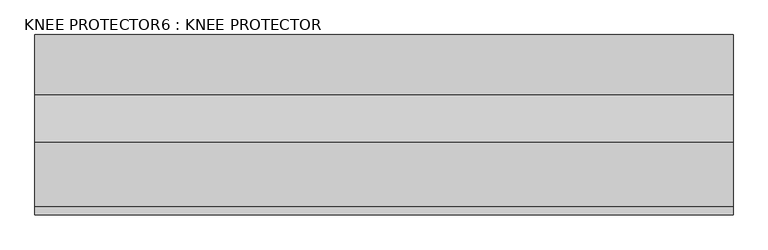
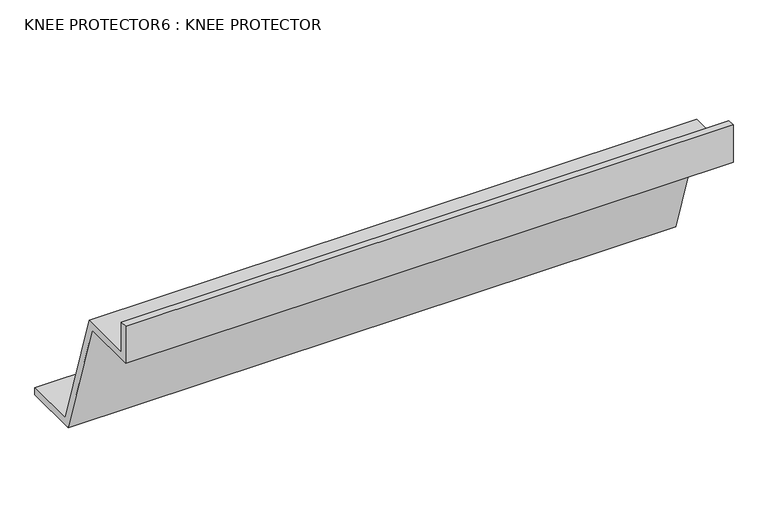
"""IFC4 building model written with IfcOpenShell, lengths in millimetres: furniture geometry, KNEE PROTECTOR6 : KNEE PROTECTOR."""

import ifcopenshell
import ifcopenshell.guid

model = None  # the IFC model being written
_history = None  # IfcOwnerHistory: only IFC2X3 demands one
_inside = {}  # id of a spatial element -> (the spatial element, [elements in it])
_under = {}  # id of a project, library or spatial element -> (it, [spatial elements below it])
_declared = {}  # id of a project -> (the project, [libraries it declares])
_typed = {}  # id of a type object -> (the type object, [elements of that type])
_made_of = {}  # id of a material, layer set ... -> (it, [elements and type objects made of it])


def new_model(schema):
    """Start an empty IFC model of exactly this schema.

    Asked for "IFC4X3", IfcOpenShell would pick the latest addendum, in which some entities
    have other attributes; the version numbers below select the first issue.
    IFC2X3 requires an IfcOwnerHistory on every rooted entity: one is made here for all.
    """
    global model, _history
    if schema == "IFC4X3":
        model = ifcopenshell.file(schema_version=(4, 3, 0, 0))
    else:
        model = ifcopenshell.file(schema=schema)
    _inside.clear()
    _under.clear()
    _declared.clear()
    _typed.clear()
    _made_of.clear()
    _history = None
    if model.schema == "IFC2X3":
        org = make("IfcOrganization", Name="unknown")
        user = make(
            "IfcPersonAndOrganization",
            ThePerson=make("IfcPerson", FamilyName="unknown"),
            TheOrganization=org,
        )
        app = make(
            "IfcApplication",
            ApplicationDeveloper=org,
            Version="unknown",
            ApplicationFullName="unknown",
            ApplicationIdentifier="unknown",
        )
        _history = make(
            "IfcOwnerHistory",
            OwningUser=user,
            OwningApplication=app,
            ChangeAction="ADDED",
            CreationDate=0,
        )
    return model


def make(cls, **values):
    """One entity of the class cls with the attributes given. An attribute that is None is left unset."""
    return model.create_entity(
        cls, **{name: value for name, value in values.items() if value is not None}
    )


def rooted(cls, **values):
    """An entity with a GlobalId (a new one), such as an element, a storey or a relation."""
    return make(cls, GlobalId=ifcopenshell.guid.new(), OwnerHistory=_history, **values)


def si_unit(unit_type, name, prefix=None):
    """IfcSIUnit, for example si_unit("LENGTHUNIT", "METRE", prefix="MILLI")."""
    return make("IfcSIUnit", UnitType=unit_type, Prefix=prefix, Name=name)


def assignment(units):
    """IfcUnitAssignment: the units of a project."""
    return None if units is None else make("IfcUnitAssignment", Units=units)


def point(xyz):
    """IfcCartesianPoint."""
    return None if xyz is None else make("IfcCartesianPoint", Coordinates=xyz)


def direction(xyz):
    """IfcDirection."""
    return None if xyz is None else make("IfcDirection", DirectionRatios=xyz)


def frame(location, z_axis=None, x_axis=None):
    """IfcAxis2Placement3D, a coordinate frame: its origin and axes. An axis left out is left unset."""
    return make(
        "IfcAxis2Placement3D",
        Location=point(location),
        Axis=direction(z_axis),
        RefDirection=direction(x_axis),
    )


def origin():
    """The frame at (0, 0, 0) with its axes left unset."""
    return frame((0.0, 0.0, 0.0))


def place(relative_to, where):
    """IfcLocalPlacement: puts the frame where relative to a parent placement (None: the world)."""
    return make(
        "IfcLocalPlacement", PlacementRelTo=relative_to, RelativePlacement=where
    )


def context(
    kind, dimensions, precision=None, world=None, true_north=None, identifier=None
):
    """IfcGeometricRepresentationContext, for example the 3D "Model" context."""
    return make(
        "IfcGeometricRepresentationContext",
        ContextIdentifier=identifier,
        ContextType=kind,
        CoordinateSpaceDimension=dimensions,
        Precision=precision,
        WorldCoordinateSystem=world,
        TrueNorth=true_north,
    )


def project(units=None, contexts=None):
    """IfcProject with its units and contexts."""
    return rooted(
        "IfcProject",
        Name="project",
        RepresentationContexts=contexts,
        UnitsInContext=assignment(units),
    )


def spatial(cls, under=None, at=None, **own):
    """A site, building, storey or space (cls), placed at a placement, below another one or the project."""
    s = rooted(cls, ObjectPlacement=at, **own)
    if under is not None:
        _under.setdefault(under.id(), (under, []))[1].append(s)
    return s


def polyline(points):
    """IfcPolyline through the points."""
    return make("IfcPolyline", Points=[point(p) for p in points])


def outline(outer, holes=None, kind="AREA"):
    """IfcArbitraryClosedProfileDef: a profile drawn as a closed curve; with holes, ...WithVoids."""
    if holes is None:
        return make("IfcArbitraryClosedProfileDef", ProfileType=kind, OuterCurve=outer)
    return make(
        "IfcArbitraryProfileDefWithVoids",
        ProfileType=kind,
        OuterCurve=outer,
        InnerCurves=holes,
    )


def extrude(swept, where, along, depth):
    """IfcExtrudedAreaSolid: the profile swept, set in the frame where, extruded along a direction by depth."""
    return make(
        "IfcExtrudedAreaSolid",
        SweptArea=swept,
        Position=where,
        ExtrudedDirection=direction(along),
        Depth=depth,
    )


def shape(context_of_items, identifier, shape_type, items):
    """IfcShapeRepresentation: the items that make up one representation, for example the "Body"."""
    return make(
        "IfcShapeRepresentation",
        ContextOfItems=context_of_items,
        RepresentationIdentifier=identifier,
        RepresentationType=shape_type,
        Items=items,
    )


def source(mapping_origin, context_of_items, identifier, shape_type, items):
    """IfcRepresentationMap: a shape defined once, which mapped items show again and again."""
    return make(
        "IfcRepresentationMap",
        MappingOrigin=mapping_origin,
        MappedRepresentation=shape(context_of_items, identifier, shape_type, items),
    )


def transform(
    local_origin,
    x_axis=None,
    y_axis=None,
    z_axis=None,
    scale=None,
    scale2=None,
    scale3=None,
    uniform=True,
):
    """IfcCartesianTransformationOperator3D, or its non-uniform kind. x_axis, y_axis, z_axis: its Axis1, 2, 3."""
    if uniform:
        return make(
            "IfcCartesianTransformationOperator3D",
            Axis1=direction(x_axis),
            Axis2=direction(y_axis),
            LocalOrigin=point(local_origin),
            Scale=scale,
            Axis3=direction(z_axis),
        )
    return make(
        "IfcCartesianTransformationOperator3DnonUniform",
        Axis1=direction(x_axis),
        Axis2=direction(y_axis),
        LocalOrigin=point(local_origin),
        Scale=scale,
        Axis3=direction(z_axis),
        Scale2=scale2,
        Scale3=scale3,
    )


def mapped(mapping_source, mapping_target):
    """IfcMappedItem: shows the shape of a source again, moved by a transform."""
    return make(
        "IfcMappedItem", MappingSource=mapping_source, MappingTarget=mapping_target
    )


def made_of(thing, what):
    """Note that an element or type object is made of a material, layer set ...; save() writes the relation."""
    if what is not None:
        _made_of.setdefault(what.id(), (what, []))[1].append(thing)
    return thing


def element(
    cls,
    number,
    at=None,
    inside=None,
    cuts=None,
    type_object=None,
    material=None,
    context=None,
    identifier="Body",
    shape_type=None,
    held_by="IfcProductDefinitionShape",
    body=None,
    shapes=None,
    **own,
):
    """One element of the class cls, such as IfcWall. Its Tag is "e" and its number.

    at: its placement. inside: the storey or other place that contains it. cuts: it is an
    opening in that element (IfcRelVoidsElement). A single representation is given by context,
    identifier, shape_type and body (its items); several are given by shapes. held_by: the class
    of the entity that holds the representations. save() writes the other relations.
    """
    e = rooted(cls, Tag="e%d" % number, ObjectPlacement=at, **own)
    if body is not None:
        shapes = [shape(context, identifier, shape_type, body)]
    if shapes is not None:
        e.Representation = make(held_by, Representations=shapes)
    if inside is not None:
        _inside.setdefault(inside.id(), (inside, []))[1].append(e)
    if cuts is not None:
        rooted(
            "IfcRelVoidsElement", RelatingBuildingElement=cuts, RelatedOpeningElement=e
        )
    if type_object is not None:
        _typed.setdefault(type_object.id(), (type_object, []))[1].append(e)
    return made_of(e, material)


def aggregate(whole, parts):
    """IfcRelAggregates: a whole, such as a stair, and the parts it consists of."""
    return rooted("IfcRelAggregates", RelatingObject=whole, RelatedObjects=parts)


def save(model, path):
    """Write the relations noted so far, then the file.

    IfcRelAggregates (storeys below a building ...), IfcRelContainedInSpatialStructure (elements
    in a storey), IfcRelDefinesByType, IfcRelAssociatesMaterial and IfcRelDeclares: one each for
    every whole, place, type object, material and project.
    """
    for whole, parts in _under.values():
        aggregate(whole, parts)
    for where, things in _inside.values():
        rooted(
            "IfcRelContainedInSpatialStructure",
            RelatedElements=things,
            RelatingStructure=where,
        )
    for kind, things in _typed.values():
        rooted("IfcRelDefinesByType", RelatedObjects=things, RelatingType=kind)
    for what, things in _made_of.values():
        rooted("IfcRelAssociatesMaterial", RelatedObjects=things, RelatingMaterial=what)
    for by, libraries in _declared.values():
        rooted("IfcRelDeclares", RelatingContext=by, RelatedDefinitions=libraries)
    model.write(path)


def knee_protector6_knee_protector_b4004326(model_context):
    return source(origin(), model_context, "Body", "SweptSolid", [
        extrude(outline(polyline([(-237028.2315414, 685.8), (-237028.2315414, 825.5), (-237002.8315414, 825.5), (-237002.8315414, 711.2), (-236803.9902606, 711.2), (-236655.4369755, 254.0), (-236469.4315414, 254.0), (-236469.4315414, 228.6), (-236673.8911557, 228.6), (-236822.4444408, 685.8), (-237028.2315414, 685.8)])), frame((-716725.3228174, 0.0, 0.0), z_axis=(1.0, 0.0, 0.0), x_axis=(0.0, 1.0, 0.0)), (0.0, 0.0, 1.0), 2162.175),
    ])


if __name__ == "__main__":
    model = new_model("IFC4")
    model_context = context("Model", 3, world=origin())
    ifc_project = project(units=[si_unit("LENGTHUNIT", "METRE", prefix="MILLI")], contexts=[model_context])
    site = spatial("IfcSite", under=ifc_project)
    building = spatial("IfcBuilding", under=site)
    placement = place(None, origin())
    knee_protector6_knee_protector_shape = knee_protector6_knee_protector_b4004326(model_context)
    element("IfcFurniture", 1, ObjectType="KNEE PROTECTOR6 : KNEE PROTECTOR", at=placement, inside=building, context=model_context, shape_type="MappedRepresentation", body=[
        mapped(knee_protector6_knee_protector_shape, transform((0.0, 0.0, 0.0), x_axis=(1.0, 0.0, 0.0), y_axis=(0.0, 1.0, 0.0), z_axis=(0.0, 0.0, 1.0))),
    ])
    save(model, "model.ifc")

# Revit data of these elements
# Element 1 (IfcFurniture, "KNEE PROTECTOR6 : KNEE PROTECTOR")
#   Materials on its faces: "CASEWORK"
# Materials
#   "CASEWORK": class "Generic", colour RGB 181 181 181, transparency 0, Cost = 0
